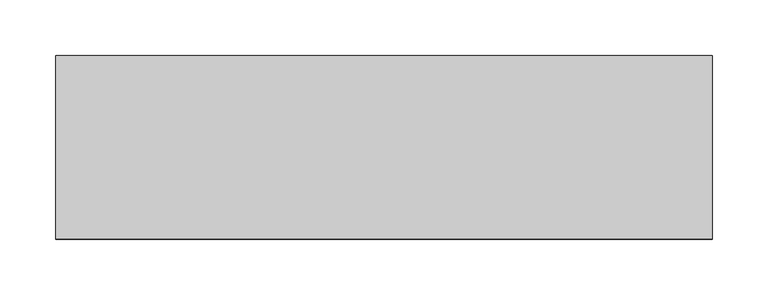
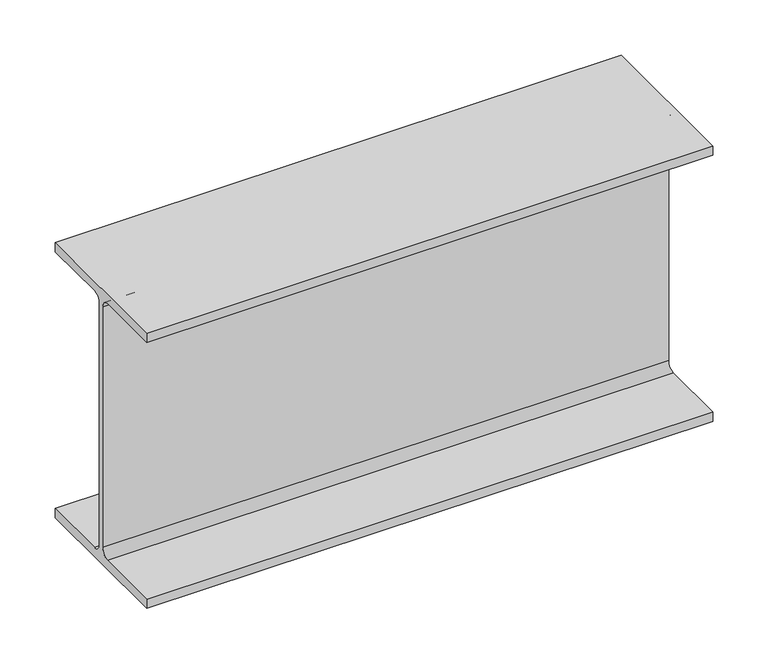
"""IFC4 building model written with IfcOpenShell, lengths in millimetres: beam geometry, Old_Steel Beam_H-KSD3502 : H_SB_ASB_H-300×150x6.5x9."""

import ifcopenshell
import ifcopenshell.guid

model = None  # the IFC model being written
_history = None  # IfcOwnerHistory: only IFC2X3 demands one
_inside = {}  # id of a spatial element -> (the spatial element, [elements in it])
_under = {}  # id of a project, library or spatial element -> (it, [spatial elements below it])
_declared = {}  # id of a project -> (the project, [libraries it declares])
_typed = {}  # id of a type object -> (the type object, [elements of that type])
_made_of = {}  # id of a material, layer set ... -> (it, [elements and type objects made of it])


def new_model(schema):
    """Start an empty IFC model of exactly this schema.

    Asked for "IFC4X3", IfcOpenShell would pick the latest addendum, in which some entities
    have other attributes; the version numbers below select the first issue.
    IFC2X3 requires an IfcOwnerHistory on every rooted entity: one is made here for all.
    """
    global model, _history
    if schema == "IFC4X3":
        model = ifcopenshell.file(schema_version=(4, 3, 0, 0))
    else:
        model = ifcopenshell.file(schema=schema)
    _inside.clear()
    _under.clear()
    _declared.clear()
    _typed.clear()
    _made_of.clear()
    _history = None
    if model.schema == "IFC2X3":
        org = make("IfcOrganization", Name="unknown")
        user = make(
            "IfcPersonAndOrganization",
            ThePerson=make("IfcPerson", FamilyName="unknown"),
            TheOrganization=org,
        )
        app = make(
            "IfcApplication",
            ApplicationDeveloper=org,
            Version="unknown",
            ApplicationFullName="unknown",
            ApplicationIdentifier="unknown",
        )
        _history = make(
            "IfcOwnerHistory",
            OwningUser=user,
            OwningApplication=app,
            ChangeAction="ADDED",
            CreationDate=0,
        )
    return model


def make(cls, **values):
    """One entity of the class cls with the attributes given. An attribute that is None is left unset."""
    return model.create_entity(
        cls, **{name: value for name, value in values.items() if value is not None}
    )


def rooted(cls, **values):
    """An entity with a GlobalId (a new one), such as an element, a storey or a relation."""
    return make(cls, GlobalId=ifcopenshell.guid.new(), OwnerHistory=_history, **values)


def si_unit(unit_type, name, prefix=None):
    """IfcSIUnit, for example si_unit("LENGTHUNIT", "METRE", prefix="MILLI")."""
    return make("IfcSIUnit", UnitType=unit_type, Prefix=prefix, Name=name)


def assignment(units):
    """IfcUnitAssignment: the units of a project."""
    return None if units is None else make("IfcUnitAssignment", Units=units)


def point(xyz):
    """IfcCartesianPoint."""
    return None if xyz is None else make("IfcCartesianPoint", Coordinates=xyz)


def direction(xyz):
    """IfcDirection."""
    return None if xyz is None else make("IfcDirection", DirectionRatios=xyz)


def frame(location, z_axis=None, x_axis=None):
    """IfcAxis2Placement3D, a coordinate frame: its origin and axes. An axis left out is left unset."""
    return make(
        "IfcAxis2Placement3D",
        Location=point(location),
        Axis=direction(z_axis),
        RefDirection=direction(x_axis),
    )


def frame_2d(location, x_axis=None):
    """IfcAxis2Placement2D, a coordinate frame in the plane: its origin and x axis."""
    return make(
        "IfcAxis2Placement2D", Location=point(location), RefDirection=direction(x_axis)
    )


def origin():
    """The frame at (0, 0, 0) with its axes left unset."""
    return frame((0.0, 0.0, 0.0))


def place(relative_to, where):
    """IfcLocalPlacement: puts the frame where relative to a parent placement (None: the world)."""
    return make(
        "IfcLocalPlacement", PlacementRelTo=relative_to, RelativePlacement=where
    )


def context(
    kind, dimensions, precision=None, world=None, true_north=None, identifier=None
):
    """IfcGeometricRepresentationContext, for example the 3D "Model" context."""
    return make(
        "IfcGeometricRepresentationContext",
        ContextIdentifier=identifier,
        ContextType=kind,
        CoordinateSpaceDimension=dimensions,
        Precision=precision,
        WorldCoordinateSystem=world,
        TrueNorth=true_north,
    )


def project(units=None, contexts=None):
    """IfcProject with its units and contexts."""
    return rooted(
        "IfcProject",
        Name="project",
        RepresentationContexts=contexts,
        UnitsInContext=assignment(units),
    )


def spatial(cls, under=None, at=None, **own):
    """A site, building, storey or space (cls), placed at a placement, below another one or the project."""
    s = rooted(cls, ObjectPlacement=at, **own)
    if under is not None:
        _under.setdefault(under.id(), (under, []))[1].append(s)
    return s


def polyline(points):
    """IfcPolyline through the points."""
    return make("IfcPolyline", Points=[point(p) for p in points])


def circle_curve(where, radius):
    """IfcCircle in the frame where."""
    return make("IfcCircle", Position=where, Radius=radius)


def trimmed(basis, trim1, trim2, sense, master):
    """IfcTrimmedCurve: the piece of a basis curve between two trims."""
    return make(
        "IfcTrimmedCurve",
        BasisCurve=basis,
        Trim1=trim1,
        Trim2=trim2,
        SenseAgreement=sense,
        MasterRepresentation=master,
    )


def segment(curve, same_sense, transition):
    """IfcCompositeCurveSegment."""
    return make(
        "IfcCompositeCurveSegment",
        Transition=transition,
        SameSense=same_sense,
        ParentCurve=curve,
    )


def composite_curve(segments, self_intersect=None):
    """IfcCompositeCurve: segments joined end to end."""
    return make("IfcCompositeCurve", Segments=segments, SelfIntersect=self_intersect)


def outline(outer, holes=None, kind="AREA"):
    """IfcArbitraryClosedProfileDef: a profile drawn as a closed curve; with holes, ...WithVoids."""
    if holes is None:
        return make("IfcArbitraryClosedProfileDef", ProfileType=kind, OuterCurve=outer)
    return make(
        "IfcArbitraryProfileDefWithVoids",
        ProfileType=kind,
        OuterCurve=outer,
        InnerCurves=holes,
    )


def extrude(swept, where, along, depth):
    """IfcExtrudedAreaSolid: the profile swept, set in the frame where, extruded along a direction by depth."""
    return make(
        "IfcExtrudedAreaSolid",
        SweptArea=swept,
        Position=where,
        ExtrudedDirection=direction(along),
        Depth=depth,
    )


def shape(context_of_items, identifier, shape_type, items):
    """IfcShapeRepresentation: the items that make up one representation, for example the "Body"."""
    return make(
        "IfcShapeRepresentation",
        ContextOfItems=context_of_items,
        RepresentationIdentifier=identifier,
        RepresentationType=shape_type,
        Items=items,
    )


def source(mapping_origin, context_of_items, identifier, shape_type, items):
    """IfcRepresentationMap: a shape defined once, which mapped items show again and again."""
    return make(
        "IfcRepresentationMap",
        MappingOrigin=mapping_origin,
        MappedRepresentation=shape(context_of_items, identifier, shape_type, items),
    )


def transform(
    local_origin,
    x_axis=None,
    y_axis=None,
    z_axis=None,
    scale=None,
    scale2=None,
    scale3=None,
    uniform=True,
):
    """IfcCartesianTransformationOperator3D, or its non-uniform kind. x_axis, y_axis, z_axis: its Axis1, 2, 3."""
    if uniform:
        return make(
            "IfcCartesianTransformationOperator3D",
            Axis1=direction(x_axis),
            Axis2=direction(y_axis),
            LocalOrigin=point(local_origin),
            Scale=scale,
            Axis3=direction(z_axis),
        )
    return make(
        "IfcCartesianTransformationOperator3DnonUniform",
        Axis1=direction(x_axis),
        Axis2=direction(y_axis),
        LocalOrigin=point(local_origin),
        Scale=scale,
        Axis3=direction(z_axis),
        Scale2=scale2,
        Scale3=scale3,
    )


def mapped(mapping_source, mapping_target):
    """IfcMappedItem: shows the shape of a source again, moved by a transform."""
    return make(
        "IfcMappedItem", MappingSource=mapping_source, MappingTarget=mapping_target
    )


def made_of(thing, what):
    """Note that an element or type object is made of a material, layer set ...; save() writes the relation."""
    if what is not None:
        _made_of.setdefault(what.id(), (what, []))[1].append(thing)
    return thing


def element(
    cls,
    number,
    at=None,
    inside=None,
    cuts=None,
    type_object=None,
    material=None,
    context=None,
    identifier="Body",
    shape_type=None,
    held_by="IfcProductDefinitionShape",
    body=None,
    shapes=None,
    **own,
):
    """One element of the class cls, such as IfcWall. Its Tag is "e" and its number.

    at: its placement. inside: the storey or other place that contains it. cuts: it is an
    opening in that element (IfcRelVoidsElement). A single representation is given by context,
    identifier, shape_type and body (its items); several are given by shapes. held_by: the class
    of the entity that holds the representations. save() writes the other relations.
    """
    e = rooted(cls, Tag="e%d" % number, ObjectPlacement=at, **own)
    if body is not None:
        shapes = [shape(context, identifier, shape_type, body)]
    if shapes is not None:
        e.Representation = make(held_by, Representations=shapes)
    if inside is not None:
        _inside.setdefault(inside.id(), (inside, []))[1].append(e)
    if cuts is not None:
        rooted(
            "IfcRelVoidsElement", RelatingBuildingElement=cuts, RelatedOpeningElement=e
        )
    if type_object is not None:
        _typed.setdefault(type_object.id(), (type_object, []))[1].append(e)
    return made_of(e, material)


def aggregate(whole, parts):
    """IfcRelAggregates: a whole, such as a stair, and the parts it consists of."""
    return rooted("IfcRelAggregates", RelatingObject=whole, RelatedObjects=parts)


def save(model, path):
    """Write the relations noted so far, then the file.

    IfcRelAggregates (storeys below a building ...), IfcRelContainedInSpatialStructure (elements
    in a storey), IfcRelDefinesByType, IfcRelAssociatesMaterial and IfcRelDeclares: one each for
    every whole, place, type object, material and project.
    """
    for whole, parts in _under.values():
        aggregate(whole, parts)
    for where, things in _inside.values():
        rooted(
            "IfcRelContainedInSpatialStructure",
            RelatedElements=things,
            RelatingStructure=where,
        )
    for kind, things in _typed.values():
        rooted("IfcRelDefinesByType", RelatedObjects=things, RelatingType=kind)
    for what, things in _made_of.values():
        rooted("IfcRelAssociatesMaterial", RelatedObjects=things, RelatingMaterial=what)
    for by, libraries in _declared.values():
        rooted("IfcRelDeclares", RelatingContext=by, RelatedDefinitions=libraries)
    model.write(path)


def beam_aae560ba(model_context):
    return source(origin(), model_context, "Body", "SweptSolid", [
        extrude(outline(composite_curve([segment(polyline([(-82.5, -141.5), (-11.9, -141.5)]), True, "CONTINUOUS"), segment(trimmed(circle_curve(frame_2d((-11.9, -132.6)), 8.9), [point((-11.9, -141.5))], [point((-3.0, -132.6))], True, "CARTESIAN"), True, "CONTINUOUS"), segment(polyline([(-3.0, -132.6), (-3.0, 132.6)]), True, "CONTINUOUS"), segment(trimmed(circle_curve(frame_2d((-11.9, 132.6)), 8.9), [point((-3.0, 132.6))], [point((-11.9, 141.5))], True, "CARTESIAN"), True, "CONTINUOUS"), segment(polyline([(-11.9, 141.5), (-82.5, 141.5), (-82.5, 151.7), (82.5, 151.7), (82.5, 141.5), (11.9, 141.5)]), True, "CONTINUOUS"), segment(trimmed(circle_curve(frame_2d((11.9, 132.6)), 8.9), [point((11.9, 141.5))], [point((3.0, 132.6))], True, "CARTESIAN"), True, "CONTINUOUS"), segment(polyline([(3.0, 132.6), (3.0, -132.6)]), True, "CONTINUOUS"), segment(trimmed(circle_curve(frame_2d((11.9, -132.6)), 8.9), [point((3.0, -132.6))], [point((11.9, -141.5))], True, "CARTESIAN"), True, "CONTINUOUS"), segment(polyline([(11.9, -141.5), (82.5, -141.5), (82.5, -151.7), (-82.5, -151.7), (-82.5, -141.5)]), True, "CONTINUOUS")], self_intersect=False)), frame((-282.3, 0.0, 0.0), z_axis=(1.0, 0.0, 0.0), x_axis=(0.0, 1.0, 0.0)), (0.0, 0.0, 1.0), 589.6),
    ])


if __name__ == "__main__":
    model = new_model("IFC4")
    model_context = context("Model", 3, world=origin())
    ifc_project = project(units=[si_unit("LENGTHUNIT", "METRE", prefix="MILLI")], contexts=[model_context])
    site = spatial("IfcSite", under=ifc_project)
    building = spatial("IfcBuilding", under=site)
    placement = place(None, origin())
    beam_shape = beam_aae560ba(model_context)
    element("IfcBeam", 1, ObjectType="Old_Steel Beam_H-KSD3502 : H_SB_ASB_H-300×150x6.5x9", at=placement, inside=building, context=model_context, shape_type="MappedRepresentation", body=[
        mapped(beam_shape, transform((0.0, 0.0, 0.0), x_axis=(1.0, 0.0, 0.0), y_axis=(0.0, 1.0, 0.0), z_axis=(0.0, 0.0, 1.0))),
    ])
    save(model, "model.ifc")

# Revit data of these elements
# Type "Old_Steel Beam_H-KSD3502 : H_SB_ASB_H-300×150x6.5x9"
#   Width = 15.0 cm
#   Web Thickness = 0.65 cm
#   Web Fillet = 1.3 cm
#   Warping Constant = 107174.0 cm⁶
#   Torsional Moment of Inertia = 9.9539 cm⁴
#   Torsional Modulus = 1.0 cm³
#   Section Area = 46.78 cm²
#   Plastic Modulus weak axis = 105.0 cm³
#   Plastic Modulus strong axis = 542.0 cm³
#   Perimeter = 1.17 m²/m
#   Nominal Weight = 36.70 kgf/m
#   Moment of Inertia weak axis = 508.00 cm⁴
#   Moment of Inertia strong axis = 7210.00 cm⁴
#   Height = 30.0 cm
#   Flange Thickness = 0.9 cm
#   Elastic Modulus weak axis = 67.7 cm³
#   Elastic Modulus strong axis = 481.0 cm³
#   Centroid Vertical = 15.0 cm
#   Centroid Horizontal = 7.5 cm
#   Length [instance default] = 1.5240 m
#   Structural Material [instance default] = Steel, 45-345
#   Assembly Code = ""
# Element 1 (IfcBeam, "Old_Steel Beam_H-KSD3502 : H_SB_ASB_H-300×150x6.5x9")
#   Structural Material = none
# Materials
#   "Steel, 45-345": class "Metal", colour RGB 189 187 185, transparency 0, Description = "Steel 345 MPa", Cost = 0
